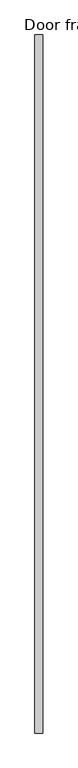
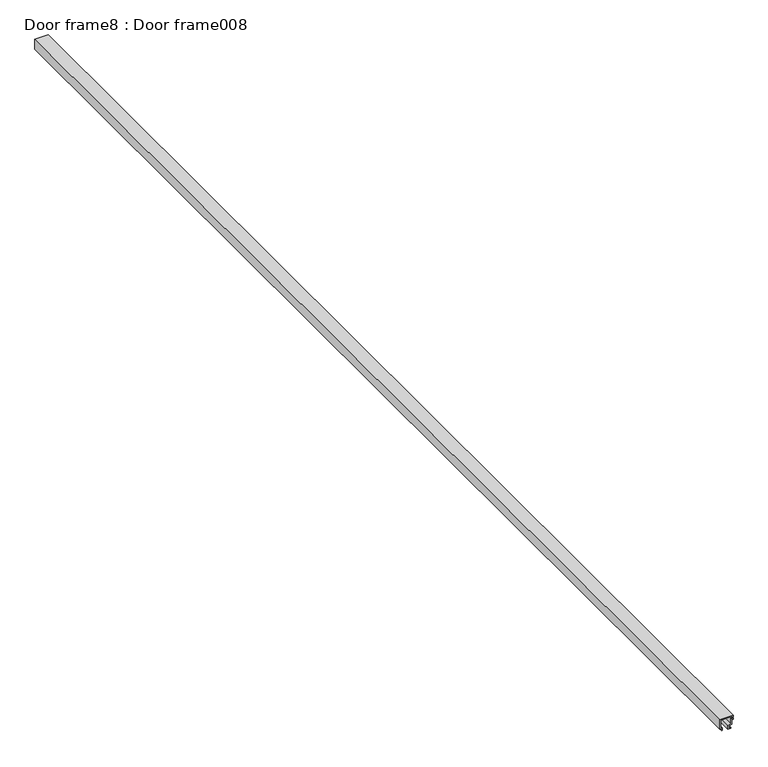
"""IFC4 building model written with IfcOpenShell, lengths in millimetres: proxy geometry, Door frame8 : Door frame008."""

from ifc_helpers import new_model, si_unit, frame, origin, place, context, project, spatial, polyline, outline, extrude, source, transform, mapped, element, save


def door_frame8_door_frame008_4371c8f4(model_context):
    return source(origin(), model_context, "Body", "SweptSolid", [
        extrude(outline(polyline([(36665.0550947, 15518.5928473), (36665.0550947, 15523.2947939), (36666.4520947, 15523.2947939), (36666.4520947, 15520.1676473), (36670.1011414, 15520.1676473), (36671.9000345, 15524.8924515), (36679.2790947, 15524.8924515), (36679.2790947, 15527.4324515), (36681.9249044, 15527.4324515), (36681.9249044, 15526.1777759), (36680.6298938, 15526.1777759), (36680.6298938, 15524.6927561), (36685.5545864, 15524.6927561), (36685.5545864, 15526.1777759), (36684.2230088, 15526.1777759), (36684.2230088, 15527.4324515), (36686.8990947, 15527.4324515), (36686.8990947, 15504.8264515), (36669.5427612, 15504.8264515), (36669.5427612, 15507.7728515), (36668.8374665, 15508.1726577), (36667.4225662, 15507.3557647), (36666.0872218, 15508.6911091), (36666.4062067, 15509.5508515), (36670.8462947, 15509.5508515), (36670.8462947, 15506.2234515), (36685.5020947, 15506.2234515), (36685.5020947, 15523.4954515), (36673.0532282, 15523.4954515), (36671.1866406, 15518.5928473), (36665.0550947, 15518.5928473)])), frame((0.0, -1052.8906567, 0.0), z_axis=(0.0, 1.0, 0.0), x_axis=(0.0, 0.0, 1.0)), (0.0, 0.0, 1.0), 1999.85),
    ])


if __name__ == "__main__":
    model = new_model("IFC4")
    model_context = context("Model", 3, world=origin())
    ifc_project = project(units=[si_unit("LENGTHUNIT", "METRE", prefix="MILLI")], contexts=[model_context])
    site = spatial("IfcSite", under=ifc_project)
    building = spatial("IfcBuilding", under=site)
    placement = place(None, origin())
    door_frame8_door_frame008_shape = door_frame8_door_frame008_4371c8f4(model_context)
    element("IfcBuildingElementProxy", 1, Name="Door frame8 : Door frame008", ObjectType="Door frame8 : Door frame008", at=placement, inside=building, context=model_context, shape_type="MappedRepresentation", body=[
        mapped(door_frame8_door_frame008_shape, transform((0.0, 0.0, 0.0), x_axis=(1.0, 0.0, 0.0), y_axis=(0.0, 1.0, 0.0), z_axis=(0.0, 0.0, 1.0))),
    ])
    save(model, "model.ifc")

# Revit data of these elements
# Type "Door frame8 : Door frame008"
#   NameOverride = "Door frame008"
# Element 1 (IfcBuildingElementProxy, "Door frame8 : Door frame008")
#   Materials on its faces: "FLEETWOOD SERIES T-3200 SINGLE SWING DOOR FRAME"
# Materials
#   "FLEETWOOD SERIES T-3200 SINGLE SWING DOOR FRAME": class "Unassigned", colour RGB 128 128 128, transparency 0, Cost = 0
